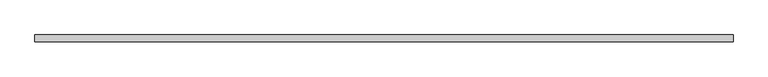
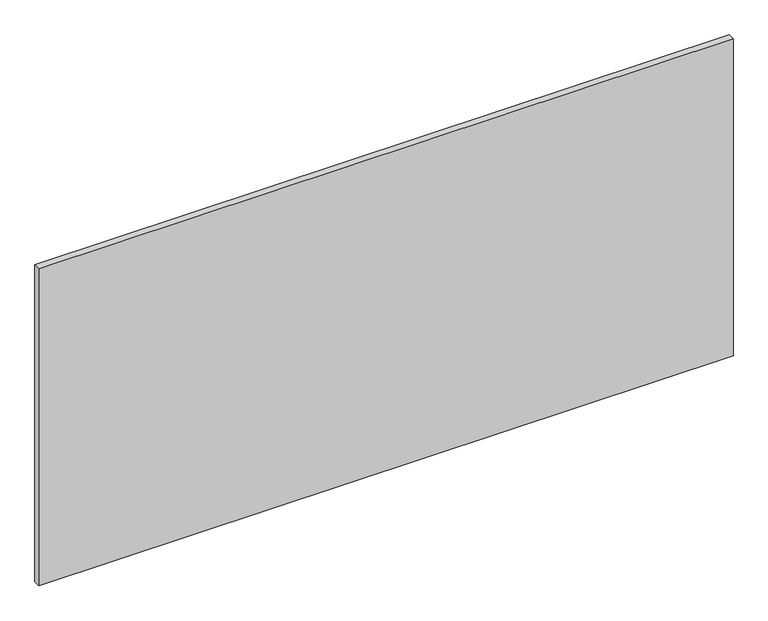
"""IFC4 building model written with IfcOpenShell, lengths in millimetres: proxy geometry, Plywood024 1176 : Plywood024 1176."""

from ifc_helpers import new_model, si_unit, frame, origin, place, context, project, spatial, polyline, outline, extrude, source, transform, mapped, element, save


def generic_models_583e60f9(model_context):
    return source(origin(), model_context, "Body", "SweptSolid", [
        extrude(outline(polyline([(3694.2883192, 9730.3383229), (3694.2883192, 9749.3851979), (5694.2883192, 9749.3851979), (5694.2883192, 9730.3383229), (3694.2883192, 9730.3383229)])), frame((0.0, 0.0, 36531.296), z_axis=(0.0, 0.0, 1.0), x_axis=(1.0, 0.0, 0.0)), (0.0, 0.0, 1.0), 965.2),
    ])


if __name__ == "__main__":
    model = new_model("IFC4")
    model_context = context("Model", 3, world=origin())
    ifc_project = project(units=[si_unit("LENGTHUNIT", "METRE", prefix="MILLI")], contexts=[model_context])
    site = spatial("IfcSite", under=ifc_project)
    building = spatial("IfcBuilding", under=site)
    placement = place(None, origin())
    generic_models_shape = generic_models_583e60f9(model_context)
    element("IfcBuildingElementProxy", 1, Name="Plywood024 1176 : Plywood024 1176", ObjectType="Plywood024 1176 : Plywood024 1176", at=placement, inside=building, context=model_context, shape_type="MappedRepresentation", body=[
        mapped(generic_models_shape, transform((0.0, 0.0, 0.0), x_axis=(1.0, 0.0, 0.0), y_axis=(0.0, 1.0, 0.0), z_axis=(0.0, 0.0, 1.0))),
    ])
    save(model, "model.ifc")

# Revit data of these elements
# Type "Plywood024 1176 : Plywood024 1176"
#   NameOverride = "Plywood024"
# Element 1 (IfcBuildingElementProxy, "Plywood024 1176 : Plywood024 1176")
#   Materials on its faces: "CDX PLYWOOD - SEE STRUCTURAL DWGS"
# Materials
#   "CDX PLYWOOD - SEE STRUCTURAL DWGS": class "Unassigned", colour RGB 177 130 114, transparency 0, Cost = 0
